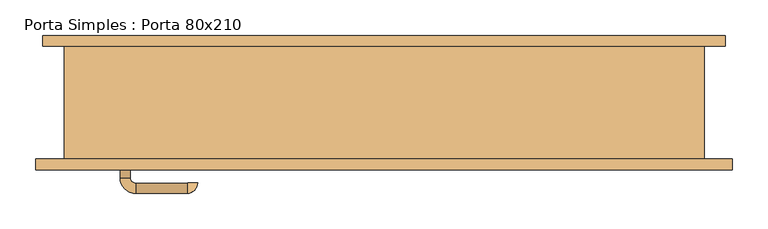
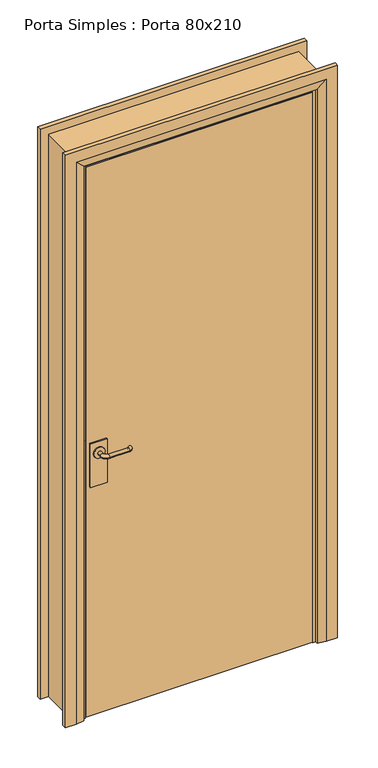
"""IFC4 building model written with IfcOpenShell, lengths in millimetres: door geometry, Porta Simples : Porta 80x210."""

from ifc_helpers import new_model, si_unit, point, frame, frame_2d, origin, place, context, project, spatial, polyline, circle_curve, ellipse_curve, trimmed, segment, composite_curve, outline, extrude, faceted_brep, source, transform, mapped, element, save
from ifc_brep_helpers import plane_surface, cylinder_surface, revolved_surface, advanced_brep


def porta_simples_porta_80x210_1d639e12(model_context):
    return source(origin(), model_context, "Body", "SolidModel", [
        extrude(outline(composite_curve([segment(trimmed(circle_curve(frame_2d((1050.0, -364.0)), 20.0), [point((1050.0, -384.0))], [point((1050.0, -344.0))], False, "CARTESIAN"), True, "CONTINUOUS"), segment(trimmed(circle_curve(frame_2d((1050.0, -364.0)), 20.0), [point((1050.0, -344.0))], [point((1050.0, -384.0))], False, "CARTESIAN"), True, "CONTINUOUS")], self_intersect=False)), frame((0.0, -38.6, 0.0), z_axis=(0.0, 1.0, 0.0), x_axis=(0.0, 0.0, 1.0)), (0.0, 0.0, 1.0), 4.5929895),
        advanced_brep(
        [(-357.0, -34.0070105, 1050.0), (-371.0, -34.0070105, 1050.0), (-357.0, -18.6, 1050.0), (-371.0, -18.6, 1050.0), (-349.0, 3.4, 1050.0), (-349.0, -10.6, 1050.0), (-277.0, -10.6, 1050.0), (-277.0, 3.4, 1050.0), (-276.0, -11.6, 1050.0), (-262.0, -11.6, 1050.0)],
        [
            (0, 1, circle_curve(frame((-364.0, -34.0070105, 1050.0), z_axis=(0.0, -1.0, 0.0), x_axis=(-1.0, 0.0, 0.0)), 7.0)),
            (1, 0, circle_curve(frame((-364.0, -34.0070105, 1050.0), z_axis=(0.0, -1.0, 0.0), x_axis=(-1.0, 0.0, 0.0)), 7.0)),
            (0, 2),
            (2, 3, circle_curve(frame((-364.0, -18.6, 1050.0), z_axis=(0.0, -1.0, 0.0), x_axis=(-1.0, 0.0, 0.0)), 7.0)),
            (3, 1),
            (3, 2, circle_curve(frame((-364.0, -18.6, 1050.0), z_axis=(0.0, -1.0, 0.0), x_axis=(-1.0, 0.0, 0.0)), 7.0)),
            (4, 3, circle_curve(frame((-349.0, -18.6, 1050.0), z_axis=(0.0, 0.0, 1.0), x_axis=(-1.0, 0.0, 0.0)), 22.0)),
            (2, 5, circle_curve(frame((-349.0, -18.6, 1050.0), z_axis=(0.0, 0.0, -1.0), x_axis=(-1.0, 0.0, 0.0)), 8.0)),
            (5, 4, circle_curve(frame((-349.0, -3.6, 1050.0), z_axis=(-1.0, 0.0, 0.0), x_axis=(0.0, 1.0, 0.0)), 7.0)),
            (4, 5, circle_curve(frame((-349.0, -3.6, 1050.0), z_axis=(-1.0, 0.0, 0.0), x_axis=(0.0, 1.0, 0.0)), 7.0)),
            (5, 6),
            (6, 7, circle_curve(frame((-277.0, -3.6, 1050.0), z_axis=(-1.0, 0.0, 0.0), x_axis=(0.0, 1.0, 0.0)), 7.0)),
            (7, 4),
            (7, 6, circle_curve(frame((-277.0, -3.6, 1050.0), z_axis=(-1.0, 0.0, 0.0), x_axis=(0.0, 1.0, 0.0)), 7.0)),
            (8, 9, circle_curve(frame((-269.0, -11.6, 1050.0), z_axis=(0.0, -1.0, 0.0), x_axis=(1.0, 0.0, 0.0)), 7.0)),
            (9, 8, circle_curve(frame((-269.0, -11.6, 1050.0), z_axis=(0.0, -1.0, 0.0), x_axis=(1.0, 0.0, 0.0)), 7.0)),
            (9, 7, circle_curve(frame((-277.0, -11.6, 1050.0), z_axis=(0.0, 0.0, 1.0), x_axis=(0.0, 1.0, 0.0)), 15.0)),
            (6, 8, circle_curve(frame((-277.0, -11.6, 1050.0), z_axis=(0.0, 0.0, -1.0), x_axis=(0.0, 1.0, 0.0)), 1.0)),
        ],
        [
            plane_surface(frame((-364.0, -34.0070105, 1050.0), z_axis=(0.0, -1.0, 0.0), x_axis=(0.0, 0.0, 1.0))),
            cylinder_surface(frame((-364.0, -34.0070105, 1050.0), z_axis=(0.0, -1.0, 0.0), x_axis=(-1.0, 0.0, 0.0)), 7.0),
            revolved_surface(trimmed(ellipse_curve(frame((-364.0, -18.6, 1050.0), z_axis=(0.0, -1.0, 0.0), x_axis=(-1.0, 0.0, 0.0)), 7.0, 7.0), [point((-357.0, -18.6, 1050.0))], [point((-371.0, -18.6, 1050.0))], True, "CARTESIAN"), (-349.0, -18.6, 1050.0), (0.0, 0.0, -1.0)),
            revolved_surface(trimmed(ellipse_curve(frame((-364.0, -18.6, 1050.0), z_axis=(0.0, -1.0, 0.0), x_axis=(-1.0, 0.0, 0.0)), 7.0, 7.0), [point((-371.0, -18.6, 1050.0))], [point((-357.0, -18.6, 1050.0))], True, "CARTESIAN"), (-349.0, -18.6, 1050.0), (0.0, 0.0, -1.0)),
            cylinder_surface(frame((-349.0, -3.6, 1050.0), z_axis=(-1.0, 0.0, 0.0), x_axis=(0.0, 1.0, 0.0)), 7.0),
            plane_surface(frame((-269.0, -11.6, 1050.0), z_axis=(0.0, -1.0, 0.0), x_axis=(0.0, 0.0, 1.0))),
            revolved_surface(trimmed(ellipse_curve(frame((-277.0, -3.6, 1050.0), z_axis=(-1.0, 0.0, 0.0), x_axis=(0.0, 1.0, 0.0)), 7.0, 7.0), [point((-277.0, -10.6, 1050.0))], [point((-277.0, 3.4, 1050.0))], True, "CARTESIAN"), (-277.0, -11.6, 1050.0), (0.0, 0.0, -1.0)),
            revolved_surface(trimmed(ellipse_curve(frame((-277.0, -3.6, 1050.0), z_axis=(-1.0, 0.0, 0.0), x_axis=(0.0, 1.0, 0.0)), 7.0, 7.0), [point((-277.0, 3.4, 1050.0))], [point((-277.0, -10.6, 1050.0))], True, "CARTESIAN"), (-277.0, -11.6, 1050.0), (0.0, 0.0, -1.0)),
        ],
        [
            (0, [[1, 2]]),
            (1, [[-1, 3, 4, 5]]),
            (1, [[-2, -5, 6, -3]]),
            (2, [[7, -4, 8, 9]]),
            (3, [[-8, -6, -7, 10]]),
            (4, [[-9, 11, 12, 13]]),
            (4, [[-10, -13, 14, -11]]),
            (5, [[15, 16]]),
            (6, [[17, -12, 18, -16]]),
            (7, [[-18, -14, -17, -15]]),
        ],
    ),
        extrude(outline(polyline([(-334.0, -44.6), (-394.0, -44.6), (-394.0, -38.6), (-334.0, -38.6), (-334.0, -44.6)])), frame((0.0, 0.0, 925.0), z_axis=(0.0, 0.0, 1.0), x_axis=(1.0, 0.0, 0.0)), (0.0, 0.0, 1.0), 165.0),
        extrude(outline(composite_curve([segment(trimmed(circle_curve(frame_2d((1050.0, -364.0)), 20.0), [point((1050.0, -384.0))], [point((1050.0, -344.0))], False, "CARTESIAN"), True, "CONTINUOUS"), segment(trimmed(circle_curve(frame_2d((1050.0, -364.0)), 20.0), [point((1050.0, -344.0))], [point((1050.0, -384.0))], False, "CARTESIAN"), True, "CONTINUOUS")], self_intersect=False)), frame((0.0, -90.1929895, 0.0), z_axis=(0.0, 1.0, 0.0), x_axis=(0.0, 0.0, 1.0)), (0.0, 0.0, 1.0), 4.5929895),
        advanced_brep(
        [(-357.0, -90.1929895, 1050.0), (-371.0, -90.1929895, 1050.0), (-371.0, -105.6, 1050.0), (-357.0, -105.6, 1050.0), (-349.0, -127.6, 1050.0), (-349.0, -113.6, 1050.0), (-277.0, -127.6, 1050.0), (-277.0, -113.6, 1050.0), (-276.0, -112.6, 1050.0), (-262.0, -112.6, 1050.0)],
        [
            (0, 1, circle_curve(frame((-364.0, -90.1929895, 1050.0), z_axis=(0.0, 1.0, 0.0), x_axis=(-1.0, 0.0, 0.0)), 7.0)),
            (1, 0, circle_curve(frame((-364.0, -90.1929895, 1050.0), z_axis=(0.0, 1.0, 0.0), x_axis=(-1.0, 0.0, 0.0)), 7.0)),
            (1, 2),
            (2, 3, circle_curve(frame((-364.0, -105.6, 1050.0), z_axis=(0.0, 1.0, 0.0), x_axis=(-1.0, 0.0, 0.0)), 7.0)),
            (3, 0),
            (3, 2, circle_curve(frame((-364.0, -105.6, 1050.0), z_axis=(0.0, 1.0, 0.0), x_axis=(-1.0, 0.0, 0.0)), 7.0)),
            (4, 5, circle_curve(frame((-349.0, -120.6, 1050.0), z_axis=(-1.0, 0.0, 0.0), x_axis=(0.0, -1.0, 0.0)), 7.0)),
            (5, 3, circle_curve(frame((-349.0, -105.6, 1050.0), z_axis=(0.0, 0.0, -1.0), x_axis=(-1.0, 0.0, 0.0)), 8.0)),
            (2, 4, circle_curve(frame((-349.0, -105.6, 1050.0), z_axis=(0.0, 0.0, 1.0), x_axis=(-1.0, 0.0, 0.0)), 22.0)),
            (5, 4, circle_curve(frame((-349.0, -120.6, 1050.0), z_axis=(-1.0, 0.0, 0.0), x_axis=(0.0, -1.0, 0.0)), 7.0)),
            (4, 6),
            (6, 7, circle_curve(frame((-277.0, -120.6, 1050.0), z_axis=(-1.0, 0.0, 0.0), x_axis=(0.0, -1.0, 0.0)), 7.0)),
            (7, 5),
            (7, 6, circle_curve(frame((-277.0, -120.6, 1050.0), z_axis=(-1.0, 0.0, 0.0), x_axis=(0.0, -1.0, 0.0)), 7.0)),
            (8, 9, circle_curve(frame((-269.0, -112.6, 1050.0), z_axis=(0.0, 1.0, 0.0), x_axis=(1.0, 0.0, 0.0)), 7.0)),
            (9, 8, circle_curve(frame((-269.0, -112.6, 1050.0), z_axis=(0.0, 1.0, 0.0), x_axis=(1.0, 0.0, 0.0)), 7.0)),
            (8, 7, circle_curve(frame((-277.0, -112.6, 1050.0), z_axis=(0.0, 0.0, -1.0), x_axis=(0.0, -1.0, 0.0)), 1.0)),
            (6, 9, circle_curve(frame((-277.0, -112.6, 1050.0), z_axis=(0.0, 0.0, 1.0), x_axis=(0.0, -1.0, 0.0)), 15.0)),
        ],
        [
            plane_surface(frame((-364.0, -90.1929895, 1050.0), z_axis=(0.0, 1.0, 0.0), x_axis=(0.0, 0.0, 1.0))),
            cylinder_surface(frame((-364.0, -90.1929895, 1050.0), z_axis=(0.0, 1.0, 0.0), x_axis=(-1.0, 0.0, 0.0)), 7.0),
            revolved_surface(trimmed(ellipse_curve(frame((-364.0, -105.6, 1050.0), z_axis=(0.0, -1.0, 0.0), x_axis=(-1.0, 0.0, 0.0)), 7.0, 7.0), [point((-357.0, -105.6, 1050.0))], [point((-371.0, -105.6, 1050.0))], True, "CARTESIAN"), (-349.0, -105.6, 1050.0), (0.0, 0.0, -1.0)),
            revolved_surface(trimmed(ellipse_curve(frame((-364.0, -105.6, 1050.0), z_axis=(0.0, -1.0, 0.0), x_axis=(-1.0, 0.0, 0.0)), 7.0, 7.0), [point((-371.0, -105.6, 1050.0))], [point((-357.0, -105.6, 1050.0))], True, "CARTESIAN"), (-349.0, -105.6, 1050.0), (0.0, 0.0, -1.0)),
            cylinder_surface(frame((-349.0, -120.6, 1050.0), z_axis=(-1.0, 0.0, 0.0), x_axis=(0.0, -1.0, 0.0)), 7.0),
            plane_surface(frame((-269.0, -112.6, 1050.0), z_axis=(0.0, 1.0, 0.0), x_axis=(0.0, 0.0, 1.0))),
            revolved_surface(trimmed(ellipse_curve(frame((-277.0, -120.6, 1050.0), z_axis=(1.0, 0.0, 0.0), x_axis=(0.0, -1.0, 0.0)), 7.0, 7.0), [point((-277.0, -113.6, 1050.0))], [point((-277.0, -127.6, 1050.0))], True, "CARTESIAN"), (-277.0, -112.6, 1050.0), (0.0, 0.0, -1.0)),
            revolved_surface(trimmed(ellipse_curve(frame((-277.0, -120.6, 1050.0), z_axis=(1.0, 0.0, 0.0), x_axis=(0.0, -1.0, 0.0)), 7.0, 7.0), [point((-277.0, -127.6, 1050.0))], [point((-277.0, -113.6, 1050.0))], True, "CARTESIAN"), (-277.0, -112.6, 1050.0), (0.0, 0.0, -1.0)),
        ],
        [
            (0, [[1, 2]]),
            (1, [[3, 4, 5, -2]]),
            (1, [[-5, 6, -3, -1]]),
            (2, [[7, 8, -4, 9]]),
            (3, [[10, -9, -6, -8]]),
            (4, [[11, 12, 13, -7]]),
            (4, [[-13, 14, -11, -10]]),
            (5, [[15, 16]]),
            (6, [[-15, 17, -12, 18]]),
            (7, [[-16, -18, -14, -17]]),
        ],
    ),
        extrude(outline(polyline([(-334.0, -79.6), (-334.0, -85.6), (-394.0, -85.6), (-394.0, -79.6), (-334.0, -79.6)])), frame((0.0, 0.0, 925.0), z_axis=(0.0, 0.0, 1.0), x_axis=(1.0, 0.0, 0.0)), (0.0, 0.0, 1.0), 165.0),
        extrude(outline(polyline([(408.0, -44.6), (408.0, -79.6), (-408.0, -79.6), (-408.0, -44.6), (408.0, -44.6)])), frame((0.0, 0.0, 53.0), z_axis=(0.0, 0.0, 1.0), x_axis=(1.0, 0.0, 0.0)), (0.0, 0.0, 1.0), 2094.0),
        faceted_brep([(480.0, 79.6, 50.0), (410.0, 79.6, 50.0), (410.0, 89.6, 50.0), (440.0, 94.6, 50.0), (480.0, 94.6, 50.0), (480.0, 94.6, 2220.0), (480.0, 79.6, 2220.0), (440.0, 94.6, 2180.0), (-440.0, 94.6, 2180.0), (-440.0, 94.6, 50.0), (-480.0, 94.6, 50.0), (-480.0, 94.6, 2220.0), (410.0, 89.6, 2150.0), (410.0, 79.6, 2150.0), (-480.0, 79.6, 2220.0), (-480.0, 79.6, 50.0), (-410.0, 79.6, 50.0), (-410.0, 79.6, 2150.0), (-410.0, 89.6, 50.0), (-410.0, 89.6, 2150.0)], [[[0, 1, 2, 3, 4]], [[4, 5, 6, 0]], [[3, 7, 8, 9, 10, 11, 5, 4]], [[2, 12, 7, 3]], [[1, 13, 12, 2]], [[0, 6, 14, 15, 16, 17, 13, 1]], [[17, 16, 18, 19]], [[15, 10, 9, 18, 16]], [[11, 10, 15, 14]], [[19, 18, 9, 8]], [[13, 17, 19, 12]], [[5, 11, 14, 6]], [[12, 19, 8, 7]]]),
        faceted_brep([(490.0, -79.6, 50.0), (490.0, -94.6, 50.0), (450.0, -94.6, 50.0), (420.0, -89.6, 50.0), (420.0, -79.6, 50.0), (420.0, -79.6, 2160.0), (-420.0, -79.6, 2160.0), (-420.0, -79.6, 50.0), (-490.0, -79.6, 50.0), (-490.0, -79.6, 2230.0), (490.0, -79.6, 2230.0), (420.0, -89.6, 2160.0), (450.0, -94.6, 2190.0), (490.0, -94.6, 2230.0), (-490.0, -94.6, 2230.0), (-490.0, -94.6, 50.0), (-450.0, -94.6, 50.0), (-450.0, -94.6, 2190.0), (-420.0, -89.6, 50.0), (-420.0, -89.6, 2160.0)], [[[0, 1, 2, 3, 4]], [[4, 5, 6, 7, 8, 9, 10, 0]], [[3, 11, 5, 4]], [[2, 12, 11, 3]], [[1, 13, 14, 15, 16, 17, 12, 2]], [[0, 10, 13, 1]], [[9, 8, 15, 14]], [[8, 7, 18, 16, 15]], [[19, 18, 7, 6]], [[17, 16, 18, 19]], [[11, 19, 6, 5]], [[10, 9, 14, 13]], [[12, 17, 19, 11]]]),
        faceted_brep([(-410.0, -79.6, 50.0), (-450.0, -79.6, 50.0), (-450.0, 79.6, 50.0), (-400.0, 79.6, 50.0), (-400.0, -42.6, 50.0), (-410.0, -42.6, 50.0), (-410.0, -42.6, 2150.0), (-410.0, -79.6, 2150.0), (-400.0, -42.6, 2140.0), (-400.0, 79.6, 2140.0), (-450.0, 79.6, 2190.0), (-450.0, -79.6, 2190.0), (410.0, -79.6, 50.0), (410.0, -42.6, 50.0), (400.0, -42.6, 50.0), (400.0, 79.6, 50.0), (450.0, 79.6, 50.0), (450.0, -79.6, 50.0), (410.0, -79.6, 2150.0), (450.0, -79.6, 2190.0), (450.0, 79.6, 2190.0), (400.0, 79.6, 2140.0), (400.0, -42.6, 2140.0), (410.0, -42.6, 2150.0)], [[[0, 1, 2, 3, 4, 5]], [[5, 6, 7, 0]], [[4, 8, 6, 5]], [[3, 9, 8, 4]], [[2, 10, 9, 3]], [[1, 11, 10, 2]], [[0, 7, 11, 1]], [[12, 13, 14, 15, 16, 17]], [[18, 12, 17, 19]], [[19, 17, 16, 20]], [[20, 16, 15, 21]], [[21, 15, 14, 22]], [[22, 14, 13, 23]], [[23, 13, 12, 18]], [[6, 23, 18, 7]], [[8, 22, 23, 6]], [[9, 21, 22, 8]], [[10, 20, 21, 9]], [[11, 19, 20, 10]], [[7, 18, 19, 11]]]),
    ])


if __name__ == "__main__":
    model = new_model("IFC4")
    model_context = context("Model", 3, world=origin())
    ifc_project = project(units=[si_unit("LENGTHUNIT", "METRE", prefix="MILLI")], contexts=[model_context])
    site = spatial("IfcSite", under=ifc_project)
    building = spatial("IfcBuilding", under=site)
    placement = place(None, origin())
    porta_simples_porta_80x210_shape = porta_simples_porta_80x210_1d639e12(model_context)
    element("IfcDoor", 1, ObjectType="Porta Simples : Porta 80x210", at=placement, inside=building, context=model_context, shape_type="MappedRepresentation", body=[
        mapped(porta_simples_porta_80x210_shape, transform((0.0, 0.0, 0.0), x_axis=(1.0, 0.0, 0.0), y_axis=(0.0, 1.0, 0.0), z_axis=(0.0, 0.0, 1.0))),
    ])
    save(model, "model.ifc")

# Revit data of these elements
# Project information
#   Project Issue Date = "Data de emissão"
#   Project Status = "Status do projeto"
#   Client Name = "Proprietário"
#   Project Address = "Insira aqui o endereço"
#   Project Name = "Nome do projeto"
#   Project Number = "0001"
# Type "Porta Simples : Porta 80x210"
#   Type Mark = "49"
#   SINAPI = ""
#   Analytic Construction = "<Nenhum>"
#   Construction Type = "300"
#   Maçaneta [instance default] = ""
#   Fechadura [instance default] = ""
#   Vão Luz (somente para informação) = 0.78 m
#   Tolerância Folha Vertical = 0.003 m
#   Módulo Básico M = 0.10 m
#   Largura de Coordenação Modular Largura CM = 0.90 m
#   Rough Width = 0.90 m
#   Deslocamento da Horizontal da Folha = 0.00 m
#   Altura de Coordenação Modular Largura CM = 2.20 m
#   Rough Height = 2.20 m
#   Altura Nominal = 2.09 m
#   Ajuste de Coordenação Topo AC Topo = 0.01 m
#   Ajuste de Coordenação Base AC Base = 0.05 m
#   Ajuste de Coordenação AC = 0.01 m
#   Tolerância Folha Horizontal = 0.002 m
#   Largura Folha (somente para informação) = 0.796 m
#   Espessura Folha = 0.035 m
#   Maçaneta - Distância da Folha = 0.044 m
#   Maçaneta - Altura = 1.00 m
#   Largura Nominal (Largura Mn) = 0.82 m
#   Distância do Nível = 0.003 m
#   Aduela Interna Espessura = 0.04 m
#   Aduela Externa Espessura = 0.05 m
#   Altura Folha (somente para informação) = 2.075 m
#   Height = 2.14 m
#   Width = 0.88 m
#   Número de Módulos Básicos nM Largura = 9
#   Número de Módulos Básicos nM Altura = 22
#   Marco Metálico = no
#   Aduela de Madeira = no
#   Aduela Metálica de Canto = no
#   Guarnição Reta = no
#   Guarnição Chanfrada = yes
#   Batente - Material [instance default] = none
#   Painel - Material [instance default] = none
#   Model = ""
#   Function = (empty or 0)
#   Description = (empty or 0)
#   Wall Closure = (empty or 0)
#   Assembly Code = ""
# Element 1 (IfcDoor, "Porta Simples : Porta 80x210")
#   Materials on its faces: "Porta - Maçaneta"
# Materials
#   "Porta - Maçaneta": class "Diversos", colour RGB 0 0 0, transparency 0
